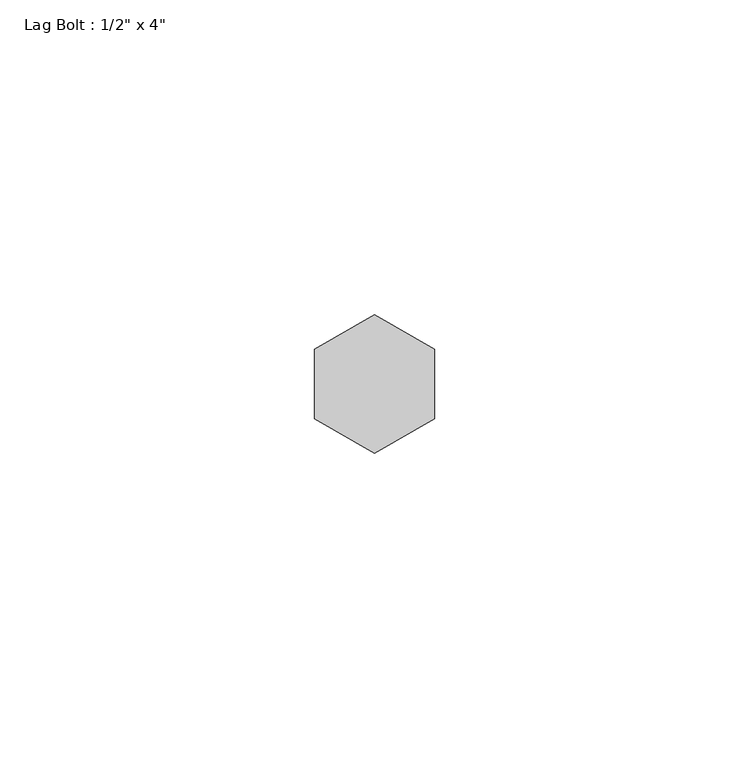
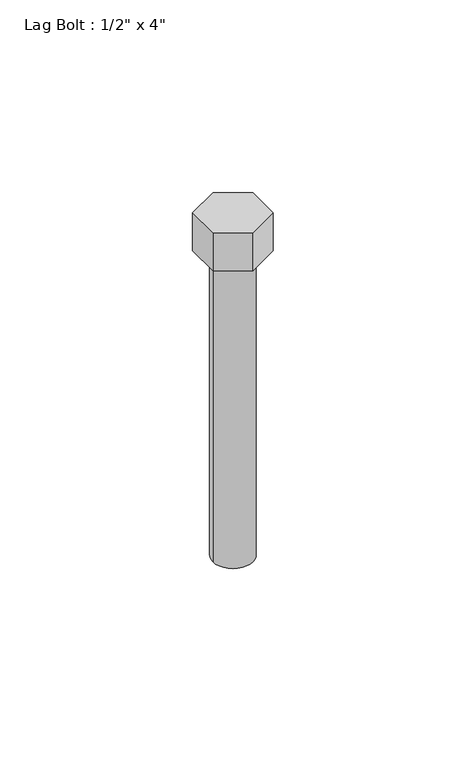
"""IFC4 building model written with IfcOpenShell, lengths in millimetres: proxy geometry."""

import ifcopenshell
import ifcopenshell.guid

model = None  # the IFC model being written
_history = None  # IfcOwnerHistory: only IFC2X3 demands one
_inside = {}  # id of a spatial element -> (the spatial element, [elements in it])
_under = {}  # id of a project, library or spatial element -> (it, [spatial elements below it])
_declared = {}  # id of a project -> (the project, [libraries it declares])
_typed = {}  # id of a type object -> (the type object, [elements of that type])
_made_of = {}  # id of a material, layer set ... -> (it, [elements and type objects made of it])


def new_model(schema):
    """Start an empty IFC model of exactly this schema.

    Asked for "IFC4X3", IfcOpenShell would pick the latest addendum, in which some entities
    have other attributes; the version numbers below select the first issue.
    IFC2X3 requires an IfcOwnerHistory on every rooted entity: one is made here for all.
    """
    global model, _history
    if schema == "IFC4X3":
        model = ifcopenshell.file(schema_version=(4, 3, 0, 0))
    else:
        model = ifcopenshell.file(schema=schema)
    _inside.clear()
    _under.clear()
    _declared.clear()
    _typed.clear()
    _made_of.clear()
    _history = None
    if model.schema == "IFC2X3":
        org = make("IfcOrganization", Name="unknown")
        user = make(
            "IfcPersonAndOrganization",
            ThePerson=make("IfcPerson", FamilyName="unknown"),
            TheOrganization=org,
        )
        app = make(
            "IfcApplication",
            ApplicationDeveloper=org,
            Version="unknown",
            ApplicationFullName="unknown",
            ApplicationIdentifier="unknown",
        )
        _history = make(
            "IfcOwnerHistory",
            OwningUser=user,
            OwningApplication=app,
            ChangeAction="ADDED",
            CreationDate=0,
        )
    return model


def make(cls, **values):
    """One entity of the class cls with the attributes given. An attribute that is None is left unset."""
    return model.create_entity(
        cls, **{name: value for name, value in values.items() if value is not None}
    )


def rooted(cls, **values):
    """An entity with a GlobalId (a new one), such as an element, a storey or a relation."""
    return make(cls, GlobalId=ifcopenshell.guid.new(), OwnerHistory=_history, **values)


def si_unit(unit_type, name, prefix=None):
    """IfcSIUnit, for example si_unit("LENGTHUNIT", "METRE", prefix="MILLI")."""
    return make("IfcSIUnit", UnitType=unit_type, Prefix=prefix, Name=name)


def assignment(units):
    """IfcUnitAssignment: the units of a project."""
    return None if units is None else make("IfcUnitAssignment", Units=units)


def point(xyz):
    """IfcCartesianPoint."""
    return None if xyz is None else make("IfcCartesianPoint", Coordinates=xyz)


def direction(xyz):
    """IfcDirection."""
    return None if xyz is None else make("IfcDirection", DirectionRatios=xyz)


def frame(location, z_axis=None, x_axis=None):
    """IfcAxis2Placement3D, a coordinate frame: its origin and axes. An axis left out is left unset."""
    return make(
        "IfcAxis2Placement3D",
        Location=point(location),
        Axis=direction(z_axis),
        RefDirection=direction(x_axis),
    )


def frame_2d(location, x_axis=None):
    """IfcAxis2Placement2D, a coordinate frame in the plane: its origin and x axis."""
    return make(
        "IfcAxis2Placement2D", Location=point(location), RefDirection=direction(x_axis)
    )


def origin():
    """The frame at (0, 0, 0) with its axes left unset."""
    return frame((0.0, 0.0, 0.0))


def origin_with_axes():
    """The frame at (0, 0, 0) with the z axis (0, 0, 1) and the x axis (1, 0, 0) written out."""
    return frame((0.0, 0.0, 0.0), z_axis=(0.0, 0.0, 1.0), x_axis=(1.0, 0.0, 0.0))


def origin_2d():
    """The frame at (0, 0) in the plane with its x axis left unset."""
    return frame_2d((0.0, 0.0))


def place(relative_to, where):
    """IfcLocalPlacement: puts the frame where relative to a parent placement (None: the world)."""
    return make(
        "IfcLocalPlacement", PlacementRelTo=relative_to, RelativePlacement=where
    )


def context(
    kind, dimensions, precision=None, world=None, true_north=None, identifier=None
):
    """IfcGeometricRepresentationContext, for example the 3D "Model" context."""
    return make(
        "IfcGeometricRepresentationContext",
        ContextIdentifier=identifier,
        ContextType=kind,
        CoordinateSpaceDimension=dimensions,
        Precision=precision,
        WorldCoordinateSystem=world,
        TrueNorth=true_north,
    )


def project(units=None, contexts=None):
    """IfcProject with its units and contexts."""
    return rooted(
        "IfcProject",
        Name="project",
        RepresentationContexts=contexts,
        UnitsInContext=assignment(units),
    )


def spatial(cls, under=None, at=None, **own):
    """A site, building, storey or space (cls), placed at a placement, below another one or the project."""
    s = rooted(cls, ObjectPlacement=at, **own)
    if under is not None:
        _under.setdefault(under.id(), (under, []))[1].append(s)
    return s


def polyline(points):
    """IfcPolyline through the points."""
    return make("IfcPolyline", Points=[point(p) for p in points])


def circle_curve(where, radius):
    """IfcCircle in the frame where."""
    return make("IfcCircle", Position=where, Radius=radius)


def trimmed(basis, trim1, trim2, sense, master):
    """IfcTrimmedCurve: the piece of a basis curve between two trims."""
    return make(
        "IfcTrimmedCurve",
        BasisCurve=basis,
        Trim1=trim1,
        Trim2=trim2,
        SenseAgreement=sense,
        MasterRepresentation=master,
    )


def segment(curve, same_sense, transition):
    """IfcCompositeCurveSegment."""
    return make(
        "IfcCompositeCurveSegment",
        Transition=transition,
        SameSense=same_sense,
        ParentCurve=curve,
    )


def composite_curve(segments, self_intersect=None):
    """IfcCompositeCurve: segments joined end to end."""
    return make("IfcCompositeCurve", Segments=segments, SelfIntersect=self_intersect)


def outline(outer, holes=None, kind="AREA"):
    """IfcArbitraryClosedProfileDef: a profile drawn as a closed curve; with holes, ...WithVoids."""
    if holes is None:
        return make("IfcArbitraryClosedProfileDef", ProfileType=kind, OuterCurve=outer)
    return make(
        "IfcArbitraryProfileDefWithVoids",
        ProfileType=kind,
        OuterCurve=outer,
        InnerCurves=holes,
    )


def extrude(swept, where, along, depth):
    """IfcExtrudedAreaSolid: the profile swept, set in the frame where, extruded along a direction by depth."""
    return make(
        "IfcExtrudedAreaSolid",
        SweptArea=swept,
        Position=where,
        ExtrudedDirection=direction(along),
        Depth=depth,
    )


def shape(context_of_items, identifier, shape_type, items):
    """IfcShapeRepresentation: the items that make up one representation, for example the "Body"."""
    return make(
        "IfcShapeRepresentation",
        ContextOfItems=context_of_items,
        RepresentationIdentifier=identifier,
        RepresentationType=shape_type,
        Items=items,
    )


def source(mapping_origin, context_of_items, identifier, shape_type, items):
    """IfcRepresentationMap: a shape defined once, which mapped items show again and again."""
    return make(
        "IfcRepresentationMap",
        MappingOrigin=mapping_origin,
        MappedRepresentation=shape(context_of_items, identifier, shape_type, items),
    )


def transform(
    local_origin,
    x_axis=None,
    y_axis=None,
    z_axis=None,
    scale=None,
    scale2=None,
    scale3=None,
    uniform=True,
):
    """IfcCartesianTransformationOperator3D, or its non-uniform kind. x_axis, y_axis, z_axis: its Axis1, 2, 3."""
    if uniform:
        return make(
            "IfcCartesianTransformationOperator3D",
            Axis1=direction(x_axis),
            Axis2=direction(y_axis),
            LocalOrigin=point(local_origin),
            Scale=scale,
            Axis3=direction(z_axis),
        )
    return make(
        "IfcCartesianTransformationOperator3DnonUniform",
        Axis1=direction(x_axis),
        Axis2=direction(y_axis),
        LocalOrigin=point(local_origin),
        Scale=scale,
        Axis3=direction(z_axis),
        Scale2=scale2,
        Scale3=scale3,
    )


def mapped(mapping_source, mapping_target):
    """IfcMappedItem: shows the shape of a source again, moved by a transform."""
    return make(
        "IfcMappedItem", MappingSource=mapping_source, MappingTarget=mapping_target
    )


def made_of(thing, what):
    """Note that an element or type object is made of a material, layer set ...; save() writes the relation."""
    if what is not None:
        _made_of.setdefault(what.id(), (what, []))[1].append(thing)
    return thing


def element(
    cls,
    number,
    at=None,
    inside=None,
    cuts=None,
    type_object=None,
    material=None,
    context=None,
    identifier="Body",
    shape_type=None,
    held_by="IfcProductDefinitionShape",
    body=None,
    shapes=None,
    **own,
):
    """One element of the class cls, such as IfcWall. Its Tag is "e" and its number.

    at: its placement. inside: the storey or other place that contains it. cuts: it is an
    opening in that element (IfcRelVoidsElement). A single representation is given by context,
    identifier, shape_type and body (its items); several are given by shapes. held_by: the class
    of the entity that holds the representations. save() writes the other relations.
    """
    e = rooted(cls, Tag="e%d" % number, ObjectPlacement=at, **own)
    if body is not None:
        shapes = [shape(context, identifier, shape_type, body)]
    if shapes is not None:
        e.Representation = make(held_by, Representations=shapes)
    if inside is not None:
        _inside.setdefault(inside.id(), (inside, []))[1].append(e)
    if cuts is not None:
        rooted(
            "IfcRelVoidsElement", RelatingBuildingElement=cuts, RelatedOpeningElement=e
        )
    if type_object is not None:
        _typed.setdefault(type_object.id(), (type_object, []))[1].append(e)
    return made_of(e, material)


def aggregate(whole, parts):
    """IfcRelAggregates: a whole, such as a stair, and the parts it consists of."""
    return rooted("IfcRelAggregates", RelatingObject=whole, RelatedObjects=parts)


def save(model, path):
    """Write the relations noted so far, then the file.

    IfcRelAggregates (storeys below a building ...), IfcRelContainedInSpatialStructure (elements
    in a storey), IfcRelDefinesByType, IfcRelAssociatesMaterial and IfcRelDeclares: one each for
    every whole, place, type object, material and project.
    """
    for whole, parts in _under.values():
        aggregate(whole, parts)
    for where, things in _inside.values():
        rooted(
            "IfcRelContainedInSpatialStructure",
            RelatedElements=things,
            RelatingStructure=where,
        )
    for kind, things in _typed.values():
        rooted("IfcRelDefinesByType", RelatedObjects=things, RelatingType=kind)
    for what, things in _made_of.values():
        rooted("IfcRelAssociatesMaterial", RelatedObjects=things, RelatingMaterial=what)
    for by, libraries in _declared.values():
        rooted("IfcRelDeclares", RelatingContext=by, RelatedDefinitions=libraries)
    model.write(path)


def proxy_b3a3e4df(model_context):
    return source(origin(), model_context, "Body", "SweptSolid", [
        extrude(outline(polyline([(-9.525, -5.4992613), (-9.525, 5.4992613), (0.0, 10.9985226), (9.525, 5.4992613), (9.525, -5.4992613), (0.0, -10.9985226), (-9.525, -5.4992613)])), origin_with_axes(), (0.0, 0.0, 1.0), 12.7),
        extrude(outline(composite_curve([segment(trimmed(circle_curve(origin_2d(), 6.35), [point((-6.35, 0.0))], [point((6.35, 0.0))], False, "CARTESIAN"), True, "CONTINUOUS"), segment(trimmed(circle_curve(origin_2d(), 6.35), [point((6.35, 0.0))], [point((-6.35, 0.0))], False, "CARTESIAN"), True, "CONTINUOUS")], self_intersect=False)), frame((0.0, 0.0, -101.6), z_axis=(0.0, 0.0, 1.0), x_axis=(1.0, 0.0, 0.0)), (0.0, 0.0, 1.0), 101.6),
    ])


if __name__ == "__main__":
    model = new_model("IFC4")
    model_context = context("Model", 3, world=origin())
    ifc_project = project(units=[si_unit("LENGTHUNIT", "METRE", prefix="MILLI")], contexts=[model_context])
    site = spatial("IfcSite", under=ifc_project)
    building = spatial("IfcBuilding", under=site)
    placement = place(None, origin())
    proxy_shape = proxy_b3a3e4df(model_context)
    element("IfcBuildingElementProxy", 1, Name="Lag Bolt : 1/2\" x 4\"", ObjectType="Lag Bolt : 1/2\" x 4\"", at=placement, inside=building, context=model_context, shape_type="MappedRepresentation", body=[
        mapped(proxy_shape, transform((0.0, 0.0, 0.0), x_axis=(1.0, 0.0, 0.0), y_axis=(0.0, 1.0, 0.0), z_axis=(0.0, 0.0, 1.0))),
    ])
    save(model, "model.ifc")

# Revit data of these elements
# Type "Lag Bolt : 1/2\" x 4\""
#   Thickness_of_Substrate [instance default] = 0' - 1"
#   Side = 0' - 0 111/256"
#   Radius = 0' - 0 1/4"
#   Length = 0' - 4"
#   Head Size = 0' - 0 3/4"
#   Head Radius = 0' - 0 3/8"
#   Head Height = 0' - 0 1/2"
#   Diameter = 0' - 0 1/2"
#   Default Elevation = 4' - 0"
#   Nut_Visibility [instance default] = no
#   Bolt Material (Size) [instance default] = none
# Element 1 (IfcBuildingElementProxy, "Lag Bolt : 1/2\" x 4\"")
#   Bolt Material (Size) = _THREADED ROD DIA 1/2" IN EPOXY - LENGTH 5" MIN
#   Materials on its faces: "_THREADED ROD DIA 1/2\" IN EPOXY - LENGTH 5\" MIN"
# Materials
#   "_THREADED ROD DIA 1/2\" IN EPOXY - LENGTH 5\" MIN": class "Generic", colour RGB 233 233 233, transparency 0, Cost = 0
